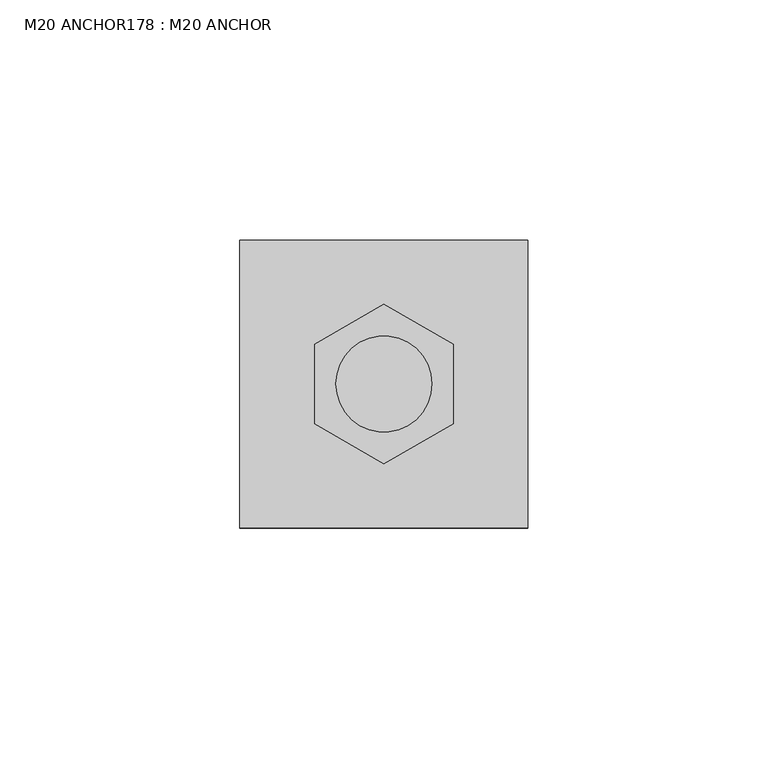
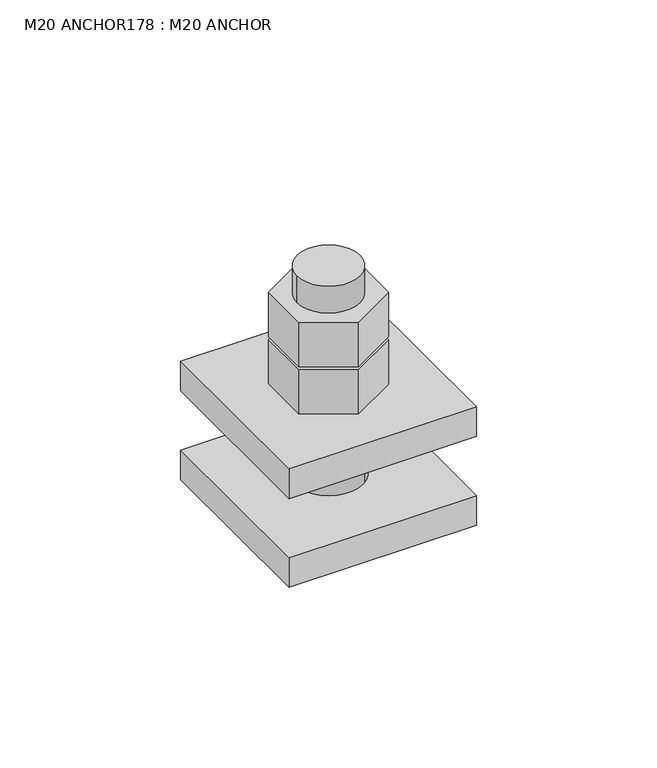
"""IFC4 building model written with IfcOpenShell, lengths in millimetres: fastener geometry, M20 ANCHOR178 : M20 ANCHOR."""

from ifc_helpers import new_model, si_unit, point, frame, frame_2d, origin, place, context, project, spatial, polyline, circle_curve, trimmed, segment, composite_curve, outline, extrude, source, transform, mapped, element, save


def m20_anchor178_m20_anchor_f42baa84(model_context):
    return source(origin(), model_context, "Body", "SweptSolid", [
        extrude(outline(polyline([(6008.0855968, 22453.9464399), (6008.0855968, 22470.5835027), (6022.4937158, 22478.9020341), (6036.9018348, 22470.5835027), (6036.9018348, 22453.9464399), (6022.4937158, 22445.6279085), (6008.0855968, 22453.9464399)]), holes=[composite_curve([segment(trimmed(circle_curve(frame_2d((6022.4937158, 22462.2649713)), 10.0), [point((6032.4937158, 22462.2649713))], [point((6012.4937158, 22462.2649713))], True, "CARTESIAN"), True, "CONTINUOUS"), segment(trimmed(circle_curve(frame_2d((6022.4937158, 22462.2649713)), 10.0), [point((6012.4937158, 22462.2649713))], [point((6032.4937158, 22462.2649713))], True, "CARTESIAN"), True, "CONTINUOUS")], self_intersect=False)]), frame((0.0, 0.0, 246.0), z_axis=(0.0, 0.0, 1.0), x_axis=(1.0, 0.0, 0.0)), (0.0, 0.0, 1.0), 15.0),
        extrude(outline(polyline([(6008.0855968, 22453.9464399), (6008.0855968, 22470.5835027), (6022.4937158, 22478.9020341), (6036.9018348, 22470.5835027), (6036.9018348, 22453.9464399), (6022.4937158, 22445.6279085), (6008.0855968, 22453.9464399)]), holes=[composite_curve([segment(trimmed(circle_curve(frame_2d((6022.4937158, 22462.2649713)), 10.0), [point((6032.4937158, 22462.2649713))], [point((6012.4937158, 22462.2649713))], True, "CARTESIAN"), True, "CONTINUOUS"), segment(trimmed(circle_curve(frame_2d((6022.4937158, 22462.2649713)), 10.0), [point((6012.4937158, 22462.2649713))], [point((6032.4937158, 22462.2649713))], True, "CARTESIAN"), True, "CONTINUOUS")], self_intersect=False)]), frame((0.0, 0.0, 230.0), z_axis=(0.0, 0.0, 1.0), x_axis=(1.0, 0.0, 0.0)), (0.0, 0.0, 1.0), 15.0),
        extrude(outline(composite_curve([segment(trimmed(circle_curve(frame_2d((6022.4937158, 22462.2649713)), 10.0), [point((6032.4937158, 22462.2649713))], [point((6012.4937158, 22462.2649713))], False, "CARTESIAN"), True, "CONTINUOUS"), segment(trimmed(circle_curve(frame_2d((6022.4937158, 22462.2649713)), 10.0), [point((6012.4937158, 22462.2649713))], [point((6032.4937158, 22462.2649713))], False, "CARTESIAN"), True, "CONTINUOUS")], self_intersect=False)), frame((0.0, 0.0, 190.0), z_axis=(0.0, 0.0, 1.0), x_axis=(1.0, 0.0, 0.0)), (0.0, 0.0, 1.0), 80.0),
        extrude(outline(polyline([(5992.4937158, 22432.2649713), (5992.4937158, 22492.2649713), (6052.4937158, 22492.2649713), (6052.4937158, 22432.2649713), (5992.4937158, 22432.2649713)]), holes=[composite_curve([segment(trimmed(circle_curve(frame_2d((6022.4937158, 22462.2649713)), 11.0), [point((6033.4937158, 22462.2649713))], [point((6011.4937158, 22462.2649713))], True, "CARTESIAN"), True, "CONTINUOUS"), segment(trimmed(circle_curve(frame_2d((6022.4937158, 22462.2649713)), 11.0), [point((6011.4937158, 22462.2649713))], [point((6033.4937158, 22462.2649713))], True, "CARTESIAN"), True, "CONTINUOUS")], self_intersect=False)]), frame((0.0, 0.0, 190.0), z_axis=(0.0, 0.0, 1.0), x_axis=(1.0, 0.0, 0.0)), (0.0, 0.0, 1.0), 10.0),
        extrude(outline(polyline([(5992.4937158, 22432.2649713), (5992.4937158, 22492.2649713), (6052.4937158, 22492.2649713), (6052.4937158, 22432.2649713), (5992.4937158, 22432.2649713)]), holes=[composite_curve([segment(trimmed(circle_curve(frame_2d((6022.4937158, 22462.2649713)), 11.0), [point((6033.4937158, 22462.2649713))], [point((6011.4937158, 22462.2649713))], True, "CARTESIAN"), True, "CONTINUOUS"), segment(trimmed(circle_curve(frame_2d((6022.4937158, 22462.2649713)), 11.0), [point((6011.4937158, 22462.2649713))], [point((6033.4937158, 22462.2649713))], True, "CARTESIAN"), True, "CONTINUOUS")], self_intersect=False)]), frame((0.0, 0.0, 220.0), z_axis=(0.0, 0.0, 1.0), x_axis=(1.0, 0.0, 0.0)), (0.0, 0.0, 1.0), 10.0),
    ])


if __name__ == "__main__":
    model = new_model("IFC4")
    model_context = context("Model", 3, world=origin())
    ifc_project = project(units=[si_unit("LENGTHUNIT", "METRE", prefix="MILLI")], contexts=[model_context])
    site = spatial("IfcSite", under=ifc_project)
    building = spatial("IfcBuilding", under=site)
    placement = place(None, origin())
    m20_anchor178_m20_anchor_shape = m20_anchor178_m20_anchor_f42baa84(model_context)
    element("IfcFastener", 1, ObjectType="M20 ANCHOR178 : M20 ANCHOR", at=placement, inside=building, context=model_context, shape_type="MappedRepresentation", body=[
        mapped(m20_anchor178_m20_anchor_shape, transform((0.0, 0.0, 0.0), x_axis=(1.0, 0.0, 0.0), y_axis=(0.0, 1.0, 0.0), z_axis=(0.0, 0.0, 1.0))),
    ])
    save(model, "model.ifc")
